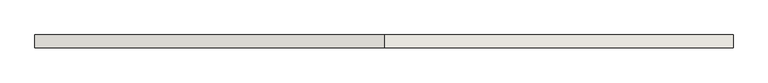
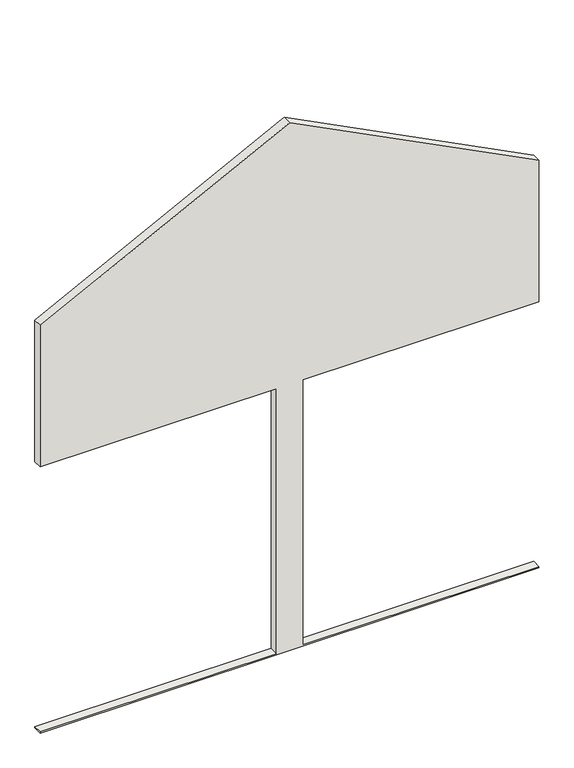
"""IFC4 building model written with IfcOpenShell, lengths in millimetres: wall geometry, 0_3d_modell."""

from ifc_helpers import new_model, si_unit, frame, origin, place, context, project, spatial, polyline, outline, extrude, source, transform, mapped, element, save


def wall_6191ee23(model_context):
    return source(origin(), model_context, "Body", "SweptSolid", [
        extrude(outline(polyline([(10.0, 3800.0), (10.0, 2000.0), (2145.0, 2000.0), (2145.0, 3800.0), (3283.5797924, 3800.0), (4251.6781465, 1900.0), (3283.5797924, 0.0), (2145.0, 0.0), (2145.0, 1800.0), (10.0, 1800.0), (10.0, 0.0), (0.0, 0.0), (0.0, 3800.0), (10.0, 3800.0)])), frame((0.0, 0.0, 0.0), z_axis=(0.0, 1.0, 0.0), x_axis=(0.0, 0.0, 1.0)), (0.0, 0.0, 1.0), 70.0),
    ])


if __name__ == "__main__":
    model = new_model("IFC4")
    model_context = context("Model", 3, world=origin())
    ifc_project = project(units=[si_unit("LENGTHUNIT", "METRE", prefix="MILLI")], contexts=[model_context])
    site = spatial("IfcSite", under=ifc_project)
    building = spatial("IfcBuilding", under=site)
    placement = place(None, origin())
    wall_shape = wall_6191ee23(model_context)
    element("IfcWall", 1, ObjectType="0_3d_modell", at=placement, inside=building, context=model_context, shape_type="MappedRepresentation", body=[
        mapped(wall_shape, transform((0.0, 0.0, 0.0), x_axis=(1.0, 0.0, 0.0), y_axis=(0.0, 1.0, 0.0), z_axis=(0.0, 0.0, 1.0))),
    ])
    save(model, "model.ifc")

# Revit data of these elements
# Element 1 (IfcWall, "0_3d_modell")
#   Materials on its faces: "Glass_Simple"
# Materials
#   "Glass_Simple": class "Unassigned", colour RGB 255 255 255, transparency 0.9
